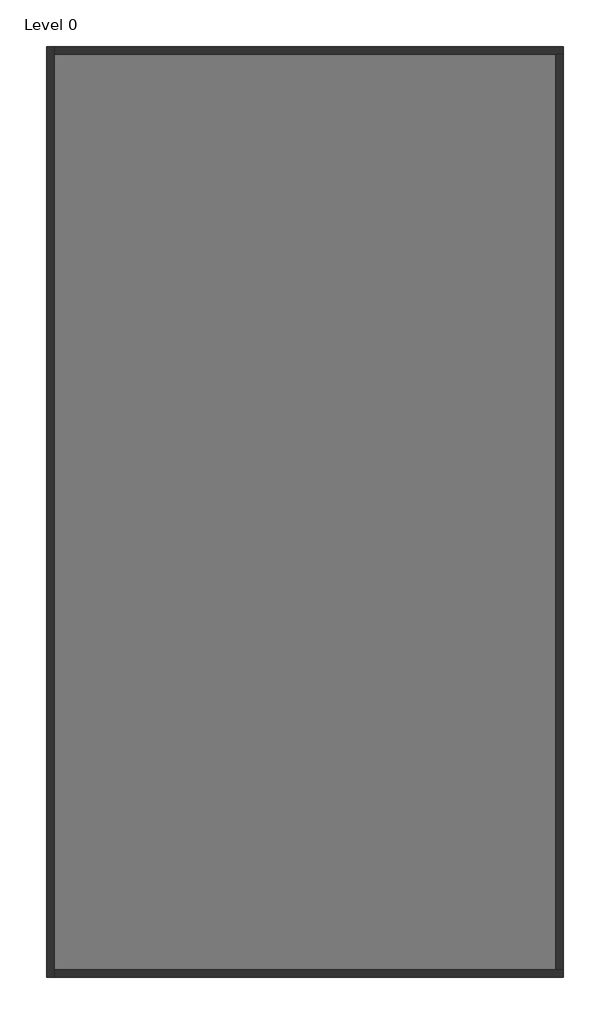
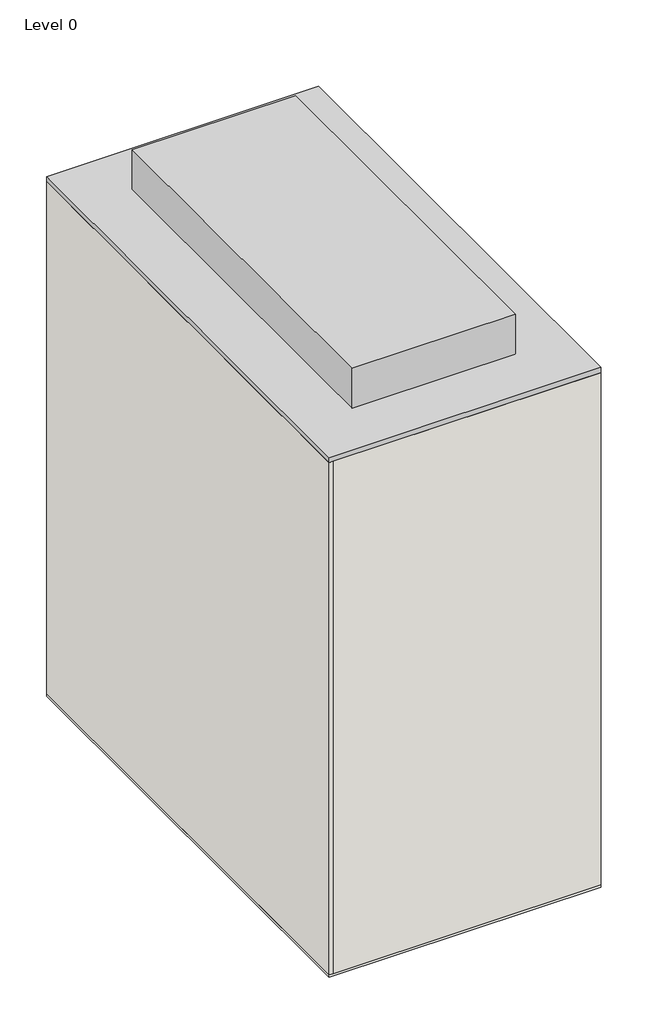
# One storey: 4 walls, 1 proxy, 1 slab.
"""IFC4 building model written with IfcOpenShell, lengths in millimetres."""

from ifc_helpers import new_model, si_unit, frame, origin, origin_with_axes, place, context, project, spatial, polyline, outline, extrude, faceted_brep, element, save

model = new_model("IFC4")

# Units and contexts
model_context = context("Model", 3, world=origin())
ifc_project = project(units=[si_unit("LENGTHUNIT", "METRE", prefix="MILLI")], contexts=[model_context])

# Site, building, storey
site = spatial("IfcSite", under=ifc_project)
building = spatial("IfcBuilding", under=site)
storey = spatial("IfcBuildingStorey", under=building, Name="Level 0", Elevation=100.0)

# Proxy
placement = place(None, origin())
element("IfcBuildingElementProxy", 1, Name="LowUrbanDensityBuilding : LowUrbanDensityBuilding", ObjectType="LowUrbanDensityBuilding : LowUrbanDensityBuilding", at=placement, inside=storey, context=model_context, shape_type="SweptSolid", body=[
    extrude(outline(polyline([(7325.2659446, 3676.2074539), (7325.2659446, -14323.7925461), (-2674.7340554, -14323.7925461), (-2674.7340554, 3676.2074539), (7325.2659446, 3676.2074539)])), origin_with_axes(), (0.0, 0.0, 1.0), 20200.0),
    extrude(outline(polyline([(5325.2659446, 1676.2074539), (5325.2659446, -12323.7925461), (-674.7340554, -12323.7925461), (-674.7340554, 1676.2074539), (5325.2659446, 1676.2074539)])), frame((0.0, 0.0, 20000.0), z_axis=(0.0, 0.0, 1.0), x_axis=(1.0, 0.0, 0.0)), (0.0, 0.0, 1.0), 1749.8),
])

# Slab
element("IfcSlab", 2, ObjectType="Floor-Concrete_100Con", at=placement, inside=storey, context=model_context, shape_type="SweptSolid", body=[
    extrude(outline(polyline([(7325.2659446, 3676.2074539), (7325.2659446, -14323.7925461), (-2674.7340554, -14323.7925461), (-2674.7340554, 3676.2074539), (7325.2659446, 3676.2074539)])), origin_with_axes(), (0.0, 0.0, 1.0), 100.0),
])

# Walls
element("IfcWall", 3, ObjectType="Wall-Ext_25Rdr-100Blk-19P", at=placement, inside=storey, context=model_context, shape_type="Brep", body=[
    faceted_brep([(-2674.7340554, 3676.2074539, 100.0), (-2674.7340554, -14323.7925461, 100.0), (-2674.7340554, -14323.7925461, 20000.0), (-2674.7340554, 3676.2074539, 20000.0), (-2530.4340554, 3676.2074539, 100.0), (-2530.4340554, 3676.2074539, 20000.0), (-2530.4340554, 3531.9074539, 20000.0), (-2530.4340554, -14179.4925461, 20000.0), (-2530.4340554, -14323.7925461, 20000.0), (-2530.4340554, -14323.7925461, 100.0), (-2530.4340554, -14179.4925461, 100.0), (-2530.4340554, 3531.9074539, 100.0)], [[[0, 1, 2, 3]], [[4, 5, 6, 7, 8, 9, 10, 11]], [[1, 0, 4, 11, 10, 9]], [[3, 2, 8, 7, 6, 5]], [[2, 1, 9, 8]], [[0, 3, 5, 4]]]),
])
element("IfcWall", 4, ObjectType="Wall-Ext_25Rdr-100Blk-19P", at=placement, inside=storey, context=model_context, shape_type="Brep", body=[
    faceted_brep([(-2530.4340554, -14323.7925461, 100.0), (7325.2659446, -14323.7925461, 100.0), (7325.2659446, -14323.7925461, 20000.0), (-2530.4340554, -14323.7925461, 20000.0), (-2530.4340554, -14179.4925461, 100.0), (-2530.4340554, -14179.4925461, 20000.0), (7180.9659446, -14179.4925461, 20000.0), (7325.2659446, -14179.4925461, 20000.0), (7325.2659446, -14179.4925461, 100.0), (7180.9659446, -14179.4925461, 100.0)], [[[0, 1, 2, 3]], [[4, 5, 6, 7, 8, 9]], [[1, 0, 4, 9, 8]], [[3, 2, 7, 6, 5]], [[0, 3, 5, 4]], [[2, 1, 8, 7]]]),
])
element("IfcWall", 5, ObjectType="Wall-Ext_25Rdr-100Blk-19P", at=placement, inside=storey, context=model_context, shape_type="Brep", body=[
    faceted_brep([(7325.2659446, 3676.2074539, 100.0), (-2530.4340554, 3676.2074539, 100.0), (-2530.4340554, 3676.2074539, 20000.0), (7325.2659446, 3676.2074539, 20000.0), (7325.2659446, 3531.9074539, 100.0), (7325.2659446, 3531.9074539, 20000.0), (7180.9659446, 3531.9074539, 20000.0), (-2530.4340554, 3531.9074539, 20000.0), (-2530.4340554, 3531.9074539, 100.0), (7180.9659446, 3531.9074539, 100.0)], [[[0, 1, 2, 3]], [[4, 5, 6, 7, 8, 9]], [[1, 0, 4, 9, 8]], [[3, 2, 7, 6, 5]], [[2, 1, 8, 7]], [[0, 3, 5, 4]]]),
])
element("IfcWall", 6, ObjectType="Wall-Ext_25Rdr-100Blk-19P", at=placement, inside=storey, context=model_context, shape_type="SweptSolid", body=[
    extrude(outline(polyline([(7325.2659446, 3531.9074539), (7325.2659446, -14179.4925461), (7180.9659446, -14179.4925461), (7180.9659446, 3531.9074539), (7325.2659446, 3531.9074539)])), frame((0.0, 0.0, 100.0), z_axis=(0.0, 0.0, 1.0), x_axis=(1.0, 0.0, 0.0)), (0.0, 0.0, 1.0), 19900.0),
])

save(model, "model.ifc")

# Revit data of these elements
# Project information
#   Project Issue Date = "Issue Date"
#   Project Status = "Project Status"
#   Client Name = "Owner"
#   Project Address = "Enter address here"
#   Project Name = "Project Name"
#   Project Number = "Project Number"
# Type "Floor-Concrete_100Con"
#   Keynote = "E60/130"
#   Function = 0
#   Layers, outside or top first: 100 mm "Concrete" (function 1)
# Type "Wall-Ext_25Rdr-100Blk-19P"
#   Keynote = "F10"
#   Layers, outside or top first: 25.3 mm "Render, Beige, Smooth" (function 5); 100 mm "Concrete Masonry Units _Low Density" (function 1); 19 mm "Plaster" (function 5)
# Element 1 (IfcBuildingElementProxy, "LowUrbanDensityBuilding : LowUrbanDensityBuilding")
#   Phase Created = New Construction
#   Materials on its faces: "Default Form"
# Element 2 (IfcSlab, "Floor-Concrete_100Con")
#   Height Offset From Level = 0 mm
#   Phase Created = New Construction
#   Materials on its faces: "Concrete"
# Element 3 (IfcWall, "Wall-Ext_25Rdr-100Blk-19P")
#   Top Offset = 0 mm
#   Base Offset = 0 mm
#   wall height = 19900 mm
#   Phase Created = New Construction
#   Base Constraint = Level 0
#   Top Constraint = Level 5
#   Materials on its faces: "Render, Beige, Smooth", "Default Wall", "Plaster"
# Elements 4, 5, 6 (IfcWall, "Wall-Ext_25Rdr-100Blk-19P")
#   Top Offset = 0 mm
#   Base Offset = 0 mm
#   wall height = 19900 mm
#   Phase Created = New Construction
#   Base Constraint = Level 0
#   Top Constraint = Level 5
#   Materials on its faces: "Default Wall", "Render, Beige, Smooth", "Plaster"
# Materials
#   "Concrete": class "Concrete", colour RGB 120 120 120, transparency 0, Description = "Portland Cement Concrete", Cost = 0
#   "Render, Beige, Smooth": class "Generic", colour RGB 213 198 180, transparency 0, Description = "physical material", Cost = 0
#   "Concrete Masonry Units _Low Density": class "Masonry", colour RGB 181 181 181, transparency 0, Description = "Concrete masonry units", Cost = 0
#   "Plaster": class "Generic", colour RGB 249 249 249, transparency 0, Description = "Plaster", Cost = 0
#   "Default Form": class "Generic", colour RGB 185 189 196, transparency 0.5, Cost = 0
#   "Default Wall": class "Miscellaneous", colour RGB 128 128 128, transparency 0, Comments = "Rendering appearance not upgraded Rendering appearance not upgraded ", Cost = 0
